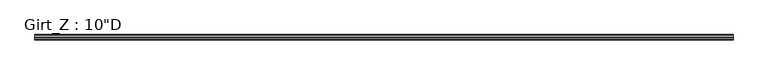
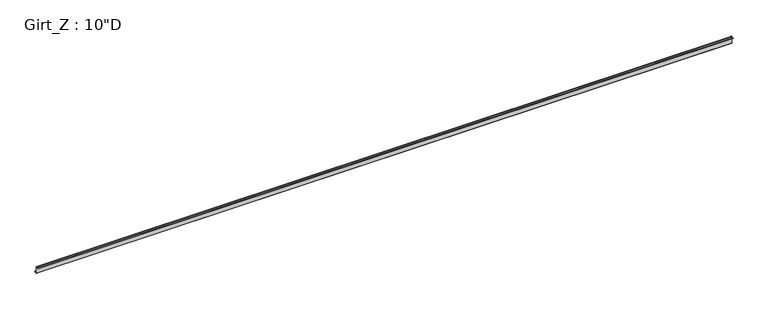
"""IFC4 building model written with IfcOpenShell, lengths in millimetres: beam geometry."""

from ifc_helpers import new_model, si_unit, point, frame, frame_2d, origin, place, context, project, spatial, polyline, circle_curve, trimmed, segment, composite_curve, outline, extrude, source, transform, mapped, element, save


def beam_08c7dc4f(model_context):
    return source(origin(), model_context, "Body", "SweptSolid", [
        extrude(outline(composite_curve([segment(polyline([(-77.9859375, 127.0), (-3.3734375, 127.0)]), True, "CONTINUOUS"), segment(trimmed(circle_curve(frame_2d((-3.3734375, 122.2375)), 4.7625), [point((-3.3734375, 127.0))], [point((1.3890625, 122.2375))], False, "CARTESIAN"), True, "CONTINUOUS"), segment(polyline([(1.3890625, 122.2375), (1.3890625, -122.2389339)]), True, "CONTINUOUS"), segment(trimmed(circle_curve(frame_2d((3.3748024, -122.2389339)), 1.9857399), [point((1.3890625, -122.2389339))], [point((3.2694106, -124.221875))], True, "CARTESIAN"), True, "CONTINUOUS"), segment(polyline([(3.2694106, -124.221875), (83.0404765, -124.221875), (94.4528742, -110.621109), (96.5810415, -112.4068534), (84.3359375, -127.0), (-1.3890625, -127.0), (-1.3890625, 122.2381931)]), True, "CONTINUOUS"), segment(trimmed(circle_curve(frame_2d((-3.3741066, 122.2381931)), 1.9850441), [point((-1.3890625, 122.2381931))], [point((-3.3005807, 124.221875))], True, "CARTESIAN"), True, "CONTINUOUS"), segment(polyline([(-3.3005807, 124.221875), (-76.6904765, 124.221875), (-88.1028742, 110.621109), (-90.2310415, 112.4068534), (-77.9859375, 127.0)]), True, "CONTINUOUS")], self_intersect=False)), frame((-12376.1500241, 0.0, 0.0), z_axis=(1.0, 0.0, 0.0), x_axis=(0.0, 1.0, 0.0)), (0.0, 0.0, 1.0), 24752.3000483),
    ])


if __name__ == "__main__":
    model = new_model("IFC4")
    model_context = context("Model", 3, world=origin())
    ifc_project = project(units=[si_unit("LENGTHUNIT", "METRE", prefix="MILLI")], contexts=[model_context])
    site = spatial("IfcSite", under=ifc_project)
    building = spatial("IfcBuilding", under=site)
    placement = place(None, origin())
    beam_shape = beam_08c7dc4f(model_context)
    element("IfcBeam", 1, ObjectType="Girt_Z : 10\"D", at=placement, inside=building, context=model_context, shape_type="MappedRepresentation", body=[
        mapped(beam_shape, transform((0.0, 0.0, 0.0), x_axis=(1.0, 0.0, 0.0), y_axis=(0.0, 1.0, 0.0), z_axis=(0.0, 0.0, 1.0))),
    ])
    save(model, "model.ifc")

# Revit data of these elements
# Type "Girt_Z : 10\"D"
#   half leg = 0' - 1 11/16"
#   Web_Thickness = 0' - 0 7/64"
#   Length [instance default] = 10' - 0"
#   Leg_2 = 0' - 3 3/8"
#   Leg_1 = 0' - 3 1/8"
#   Height = 0' - 10"
#   Structural Material [instance default] = none
# Element 1 (IfcBeam, "Girt_Z : 10\"D")
#   Structural Material = STRUCTURAL STEEL - SEE STRUCT. DWGS
#   Materials on its faces: "STRUCTURAL STEEL - SEE STRUCT. DWGS"
# Materials
#   "STRUCTURAL STEEL - SEE STRUCT. DWGS": class "Metal", colour RGB 137 146 153, transparency 0, Description = "Steel, mill finish", Cost = 0
